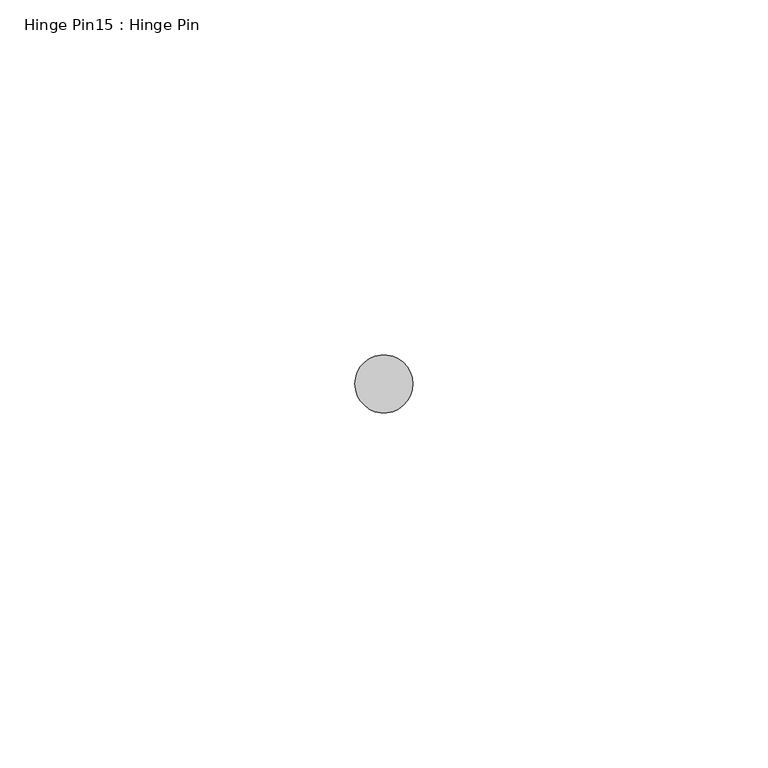
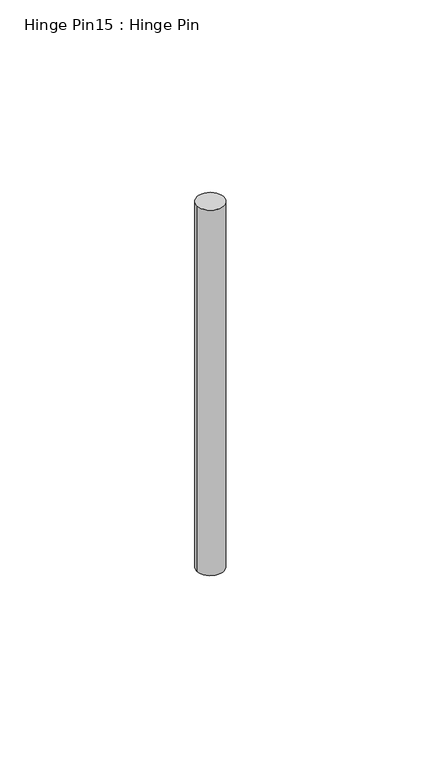
"""IFC4 building model written with IfcOpenShell, lengths in millimetres: proxy geometry, Hinge Pin15 : Hinge Pin."""

from ifc_helpers import new_model, si_unit, point, frame, frame_2d, origin, place, context, project, spatial, circle_curve, trimmed, segment, composite_curve, outline, extrude, source, transform, mapped, element, save


def hinge_pin15_hinge_pin_38e29aa4(model_context):
    return source(origin(), model_context, "Body", "SweptSolid", [
        extrude(outline(composite_curve([segment(trimmed(circle_curve(frame_2d((587319.1320739, -533984.6777841)), 4.0894), [point((587315.0426739, -533984.6777841))], [point((587323.2214739, -533984.6777841))], False, "CARTESIAN"), True, "CONTINUOUS"), segment(trimmed(circle_curve(frame_2d((587319.1320739, -533984.6777841)), 4.0894), [point((587323.2214739, -533984.6777841))], [point((587315.0426739, -533984.6777841))], False, "CARTESIAN"), True, "CONTINUOUS")], self_intersect=False)), frame((0.0, 0.0, 315.7140625), z_axis=(0.0, 0.0, 1.0), x_axis=(1.0, 0.0, 0.0)), (0.0, 0.0, 1.0), 117.871875),
    ])


if __name__ == "__main__":
    model = new_model("IFC4")
    model_context = context("Model", 3, world=origin())
    ifc_project = project(units=[si_unit("LENGTHUNIT", "METRE", prefix="MILLI")], contexts=[model_context])
    site = spatial("IfcSite", under=ifc_project)
    building = spatial("IfcBuilding", under=site)
    placement = place(None, origin())
    hinge_pin15_hinge_pin_shape = hinge_pin15_hinge_pin_38e29aa4(model_context)
    element("IfcBuildingElementProxy", 1, Name="Hinge Pin15 : Hinge Pin", ObjectType="Hinge Pin15 : Hinge Pin", at=placement, inside=building, context=model_context, shape_type="MappedRepresentation", body=[
        mapped(hinge_pin15_hinge_pin_shape, transform((0.0, 0.0, 0.0), x_axis=(1.0, 0.0, 0.0), y_axis=(0.0, 1.0, 0.0), z_axis=(0.0, 0.0, 1.0))),
    ])
    save(model, "model.ifc")

# Revit data of these elements
# Element 1 (IfcBuildingElementProxy, "Hinge Pin15 : Hinge Pin")
#   Materials on its faces: "6\"X6\" WELD-ON STL BUTT HINGE"
# Materials
#   "6\"X6\" WELD-ON STL BUTT HINGE": class "Metal", colour RGB 189 187 185, transparency 0, Description = "Carbon steel", Cost = 0
